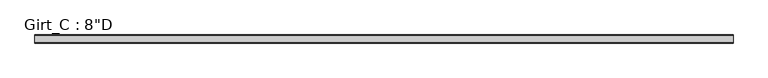
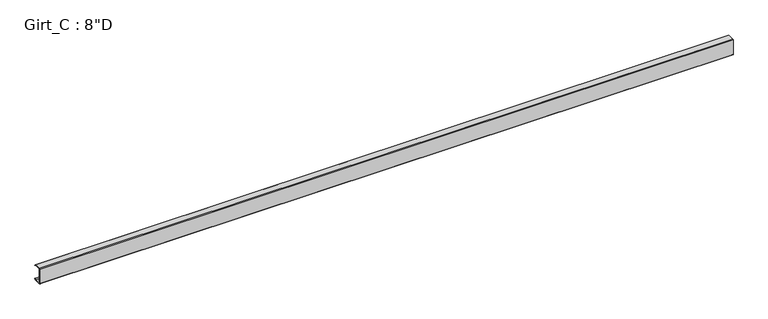
"""IFC4 building model written with IfcOpenShell, lengths in millimetres: beam geometry."""

from ifc_helpers import new_model, si_unit, point, frame, frame_2d, origin, place, context, project, spatial, polyline, circle_curve, trimmed, segment, composite_curve, outline, extrude, source, transform, mapped, element, save


def beam_e26b36c5(model_context):
    return source(origin(), model_context, "Body", "SweptSolid", [
        extrude(outline(composite_curve([segment(polyline([(87.5109375, 101.6), (99.7560415, 87.0068534), (97.6278742, 85.221109), (86.2154765, 98.821875), (3.3005807, 98.821875)]), True, "CONTINUOUS"), segment(trimmed(circle_curve(frame_2d((3.3741066, 96.8381931)), 1.9850441), [point((3.3005807, 98.821875))], [point((1.3890625, 96.8381931))], True, "CARTESIAN"), True, "CONTINUOUS"), segment(polyline([(1.3890625, 96.8381931), (1.3890625, -96.8389339)]), True, "CONTINUOUS"), segment(trimmed(circle_curve(frame_2d((3.3748024, -96.8389339)), 1.9857399), [point((1.3890625, -96.8389339))], [point((3.2694106, -98.821875))], True, "CARTESIAN"), True, "CONTINUOUS"), segment(polyline([(3.2694106, -98.821875), (86.2154765, -98.821875), (97.6510975, -85.1934327), (99.7792647, -86.979177), (87.5109375, -101.6), (3.3734375, -101.6)]), True, "CONTINUOUS"), segment(trimmed(circle_curve(frame_2d((3.3734375, -96.8375)), 4.7625), [point((3.3734375, -101.6))], [point((-1.3890625, -96.8375))], False, "CARTESIAN"), True, "CONTINUOUS"), segment(polyline([(-1.3890625, -96.8375), (-1.3890625, 96.8375)]), True, "CONTINUOUS"), segment(trimmed(circle_curve(frame_2d((3.3734375, 96.8375)), 4.7625), [point((-1.3890625, 96.8375))], [point((3.3734375, 101.6))], False, "CARTESIAN"), True, "CONTINUOUS"), segment(polyline([(3.3734375, 101.6), (87.5109375, 101.6)]), True, "CONTINUOUS")], self_intersect=False)), frame((-4340.225, 0.0, 0.0), z_axis=(1.0, 0.0, 0.0), x_axis=(0.0, 1.0, 0.0)), (0.0, 0.0, 1.0), 8680.45),
    ])


if __name__ == "__main__":
    model = new_model("IFC4")
    model_context = context("Model", 3, world=origin())
    ifc_project = project(units=[si_unit("LENGTHUNIT", "METRE", prefix="MILLI")], contexts=[model_context])
    site = spatial("IfcSite", under=ifc_project)
    building = spatial("IfcBuilding", under=site)
    placement = place(None, origin())
    beam_shape = beam_e26b36c5(model_context)
    element("IfcBeam", 1, ObjectType="Girt_C : 8\"D", at=placement, inside=building, context=model_context, shape_type="MappedRepresentation", body=[
        mapped(beam_shape, transform((0.0, 0.0, 0.0), x_axis=(1.0, 0.0, 0.0), y_axis=(0.0, 1.0, 0.0), z_axis=(0.0, 0.0, 1.0))),
    ])
    save(model, "model.ifc")

# Revit data of these elements
# Type "Girt_C : 8\"D"
#   half leg = 0' - 1 3/4"
#   Web_Thickness = 0' - 0 7/64"
#   Length [instance default] = 10' - 0"
#   Leg_1 = 0' - 3 1/2"
#   Height = 0' - 8"
#   Structural Material [instance default] = none
# Element 1 (IfcBeam, "Girt_C : 8\"D")
#   Structural Material = GALVANIZED 'CEE' SECTION (8.0x3.5C - SEE STRUCT. DWGS)
#   Materials on its faces: "GALVANIZED 'CEE' SECTION (8.0x3.5C - SEE STRUCT. DWGS)"
# Materials
#   "GALVANIZED 'CEE' SECTION (8.0x3.5C - SEE STRUCT. DWGS)": class "Metal", colour RGB 137 146 153, transparency 0, Description = "Steel, mill finish", Cost = 0
